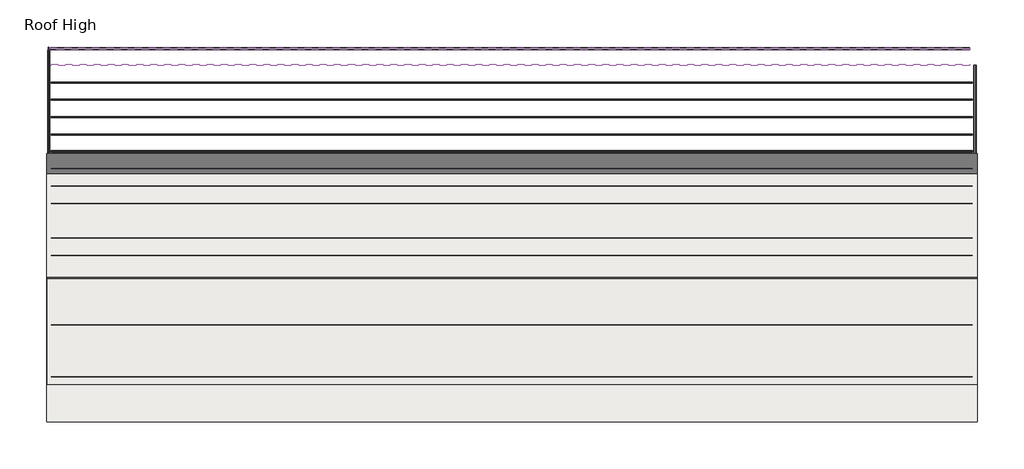
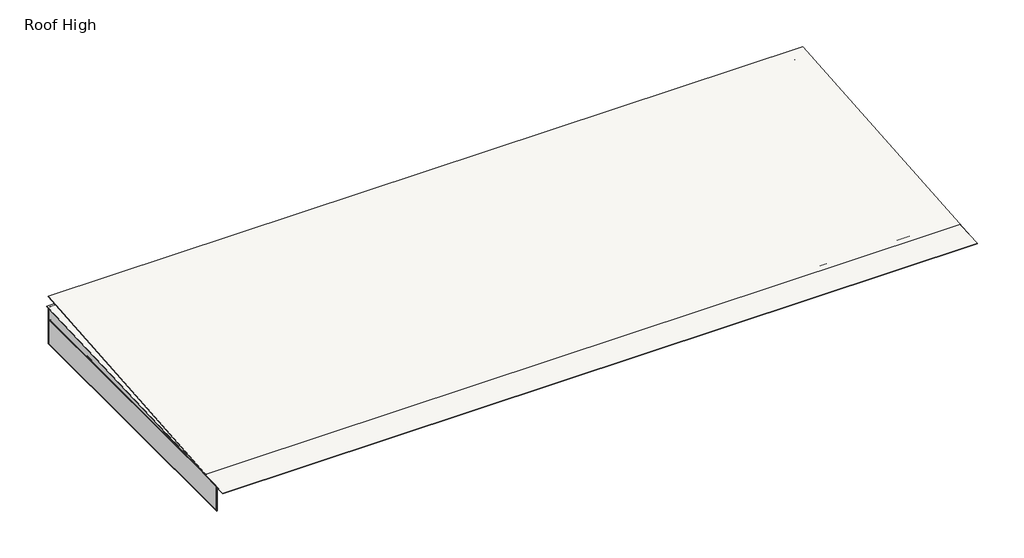
# One storey: 23 beams, 4 members, 2 roofs, 1 plate.
"""IFC4 building model written with IfcOpenShell, lengths in millimetres."""

import ifcopenshell
import ifcopenshell.guid

model = None  # the IFC model being written
_history = None  # IfcOwnerHistory: only IFC2X3 demands one
_inside = {}  # id of a spatial element -> (the spatial element, [elements in it])
_under = {}  # id of a project, library or spatial element -> (it, [spatial elements below it])
_declared = {}  # id of a project -> (the project, [libraries it declares])
_typed = {}  # id of a type object -> (the type object, [elements of that type])
_made_of = {}  # id of a material, layer set ... -> (it, [elements and type objects made of it])


def new_model(schema):
    """Start an empty IFC model of exactly this schema.

    Asked for "IFC4X3", IfcOpenShell would pick the latest addendum, in which some entities
    have other attributes; the version numbers below select the first issue.
    IFC2X3 requires an IfcOwnerHistory on every rooted entity: one is made here for all.
    """
    global model, _history
    if schema == "IFC4X3":
        model = ifcopenshell.file(schema_version=(4, 3, 0, 0))
    else:
        model = ifcopenshell.file(schema=schema)
    _inside.clear()
    _under.clear()
    _declared.clear()
    _typed.clear()
    _made_of.clear()
    _history = None
    if model.schema == "IFC2X3":
        org = make("IfcOrganization", Name="unknown")
        user = make(
            "IfcPersonAndOrganization",
            ThePerson=make("IfcPerson", FamilyName="unknown"),
            TheOrganization=org,
        )
        app = make(
            "IfcApplication",
            ApplicationDeveloper=org,
            Version="unknown",
            ApplicationFullName="unknown",
            ApplicationIdentifier="unknown",
        )
        _history = make(
            "IfcOwnerHistory",
            OwningUser=user,
            OwningApplication=app,
            ChangeAction="ADDED",
            CreationDate=0,
        )
    return model


def make(cls, **values):
    """One entity of the class cls with the attributes given. An attribute that is None is left unset."""
    return model.create_entity(
        cls, **{name: value for name, value in values.items() if value is not None}
    )


def rooted(cls, **values):
    """An entity with a GlobalId (a new one), such as an element, a storey or a relation."""
    return make(cls, GlobalId=ifcopenshell.guid.new(), OwnerHistory=_history, **values)


def si_unit(unit_type, name, prefix=None):
    """IfcSIUnit, for example si_unit("LENGTHUNIT", "METRE", prefix="MILLI")."""
    return make("IfcSIUnit", UnitType=unit_type, Prefix=prefix, Name=name)


def assignment(units):
    """IfcUnitAssignment: the units of a project."""
    return None if units is None else make("IfcUnitAssignment", Units=units)


def point(xyz):
    """IfcCartesianPoint."""
    return None if xyz is None else make("IfcCartesianPoint", Coordinates=xyz)


def direction(xyz):
    """IfcDirection."""
    return None if xyz is None else make("IfcDirection", DirectionRatios=xyz)


def frame(location, z_axis=None, x_axis=None):
    """IfcAxis2Placement3D, a coordinate frame: its origin and axes. An axis left out is left unset."""
    return make(
        "IfcAxis2Placement3D",
        Location=point(location),
        Axis=direction(z_axis),
        RefDirection=direction(x_axis),
    )


def frame_2d(location, x_axis=None):
    """IfcAxis2Placement2D, a coordinate frame in the plane: its origin and x axis."""
    return make(
        "IfcAxis2Placement2D", Location=point(location), RefDirection=direction(x_axis)
    )


def origin():
    """The frame at (0, 0, 0) with its axes left unset."""
    return frame((0.0, 0.0, 0.0))


def place(relative_to, where):
    """IfcLocalPlacement: puts the frame where relative to a parent placement (None: the world)."""
    return make(
        "IfcLocalPlacement", PlacementRelTo=relative_to, RelativePlacement=where
    )


def context(
    kind, dimensions, precision=None, world=None, true_north=None, identifier=None
):
    """IfcGeometricRepresentationContext, for example the 3D "Model" context."""
    return make(
        "IfcGeometricRepresentationContext",
        ContextIdentifier=identifier,
        ContextType=kind,
        CoordinateSpaceDimension=dimensions,
        Precision=precision,
        WorldCoordinateSystem=world,
        TrueNorth=true_north,
    )


def project(units=None, contexts=None):
    """IfcProject with its units and contexts."""
    return rooted(
        "IfcProject",
        Name="project",
        RepresentationContexts=contexts,
        UnitsInContext=assignment(units),
    )


def spatial(cls, under=None, at=None, **own):
    """A site, building, storey or space (cls), placed at a placement, below another one or the project."""
    s = rooted(cls, ObjectPlacement=at, **own)
    if under is not None:
        _under.setdefault(under.id(), (under, []))[1].append(s)
    return s


def polyline(points):
    """IfcPolyline through the points."""
    return make("IfcPolyline", Points=[point(p) for p in points])


def circle_curve(where, radius):
    """IfcCircle in the frame where."""
    return make("IfcCircle", Position=where, Radius=radius)


def trimmed(basis, trim1, trim2, sense, master):
    """IfcTrimmedCurve: the piece of a basis curve between two trims."""
    return make(
        "IfcTrimmedCurve",
        BasisCurve=basis,
        Trim1=trim1,
        Trim2=trim2,
        SenseAgreement=sense,
        MasterRepresentation=master,
    )


def segment(curve, same_sense, transition):
    """IfcCompositeCurveSegment."""
    return make(
        "IfcCompositeCurveSegment",
        Transition=transition,
        SameSense=same_sense,
        ParentCurve=curve,
    )


def composite_curve(segments, self_intersect=None):
    """IfcCompositeCurve: segments joined end to end."""
    return make("IfcCompositeCurve", Segments=segments, SelfIntersect=self_intersect)


def outline(outer, holes=None, kind="AREA"):
    """IfcArbitraryClosedProfileDef: a profile drawn as a closed curve; with holes, ...WithVoids."""
    if holes is None:
        return make("IfcArbitraryClosedProfileDef", ProfileType=kind, OuterCurve=outer)
    return make(
        "IfcArbitraryProfileDefWithVoids",
        ProfileType=kind,
        OuterCurve=outer,
        InnerCurves=holes,
    )


def extrude(swept, where, along, depth):
    """IfcExtrudedAreaSolid: the profile swept, set in the frame where, extruded along a direction by depth."""
    return make(
        "IfcExtrudedAreaSolid",
        SweptArea=swept,
        Position=where,
        ExtrudedDirection=direction(along),
        Depth=depth,
    )


def faces_of(points, faces, orient=None, outer=None):
    """IfcFace entities. A face is a list of loops; a loop is a list of indices into points, from 0.

    orient and outer hold one flag for each loop. By default every Orientation is true, the
    first loop of a face is its IfcFaceOuterBound and the others are IfcFaceBound.
    """
    made = []
    for i, loops in enumerate(faces):
        bounds = []
        for j, loop in enumerate(loops):
            is_outer = j == 0 if outer is None else outer[i][j]
            bounds.append(
                make(
                    "IfcFaceOuterBound" if is_outer else "IfcFaceBound",
                    Bound=make("IfcPolyLoop", Polygon=[points[k] for k in loop]),
                    Orientation=True if orient is None else orient[i][j],
                )
            )
        made.append(make("IfcFace", Bounds=bounds))
    return made


def faceted_brep(points, faces, orient=None, outer=None, voids=None):
    """IfcFacetedBrep: a solid bounded by flat faces; with voids (closed shells), ...WithVoids."""
    shared = [point(p) for p in points]
    hull = make("IfcClosedShell", CfsFaces=faces_of(shared, faces, orient, outer))
    if voids is None:
        return make("IfcFacetedBrep", Outer=hull)
    return make(
        "IfcFacetedBrepWithVoids",
        Outer=hull,
        Voids=[
            make(cls, CfsFaces=faces_of(shared, fs, o, b)) for cls, fs, o, b in voids
        ],
    )


def shape(context_of_items, identifier, shape_type, items):
    """IfcShapeRepresentation: the items that make up one representation, for example the "Body"."""
    return make(
        "IfcShapeRepresentation",
        ContextOfItems=context_of_items,
        RepresentationIdentifier=identifier,
        RepresentationType=shape_type,
        Items=items,
    )


def source(mapping_origin, context_of_items, identifier, shape_type, items):
    """IfcRepresentationMap: a shape defined once, which mapped items show again and again."""
    return make(
        "IfcRepresentationMap",
        MappingOrigin=mapping_origin,
        MappedRepresentation=shape(context_of_items, identifier, shape_type, items),
    )


def transform(
    local_origin,
    x_axis=None,
    y_axis=None,
    z_axis=None,
    scale=None,
    scale2=None,
    scale3=None,
    uniform=True,
):
    """IfcCartesianTransformationOperator3D, or its non-uniform kind. x_axis, y_axis, z_axis: its Axis1, 2, 3."""
    if uniform:
        return make(
            "IfcCartesianTransformationOperator3D",
            Axis1=direction(x_axis),
            Axis2=direction(y_axis),
            LocalOrigin=point(local_origin),
            Scale=scale,
            Axis3=direction(z_axis),
        )
    return make(
        "IfcCartesianTransformationOperator3DnonUniform",
        Axis1=direction(x_axis),
        Axis2=direction(y_axis),
        LocalOrigin=point(local_origin),
        Scale=scale,
        Axis3=direction(z_axis),
        Scale2=scale2,
        Scale3=scale3,
    )


def mapped(mapping_source, mapping_target):
    """IfcMappedItem: shows the shape of a source again, moved by a transform."""
    return make(
        "IfcMappedItem", MappingSource=mapping_source, MappingTarget=mapping_target
    )


def made_of(thing, what):
    """Note that an element or type object is made of a material, layer set ...; save() writes the relation."""
    if what is not None:
        _made_of.setdefault(what.id(), (what, []))[1].append(thing)
    return thing


def element(
    cls,
    number,
    at=None,
    inside=None,
    cuts=None,
    type_object=None,
    material=None,
    context=None,
    identifier="Body",
    shape_type=None,
    held_by="IfcProductDefinitionShape",
    body=None,
    shapes=None,
    **own,
):
    """One element of the class cls, such as IfcWall. Its Tag is "e" and its number.

    at: its placement. inside: the storey or other place that contains it. cuts: it is an
    opening in that element (IfcRelVoidsElement). A single representation is given by context,
    identifier, shape_type and body (its items); several are given by shapes. held_by: the class
    of the entity that holds the representations. save() writes the other relations.
    """
    e = rooted(cls, Tag="e%d" % number, ObjectPlacement=at, **own)
    if body is not None:
        shapes = [shape(context, identifier, shape_type, body)]
    if shapes is not None:
        e.Representation = make(held_by, Representations=shapes)
    if inside is not None:
        _inside.setdefault(inside.id(), (inside, []))[1].append(e)
    if cuts is not None:
        rooted(
            "IfcRelVoidsElement", RelatingBuildingElement=cuts, RelatedOpeningElement=e
        )
    if type_object is not None:
        _typed.setdefault(type_object.id(), (type_object, []))[1].append(e)
    return made_of(e, material)


def aggregate(whole, parts):
    """IfcRelAggregates: a whole, such as a stair, and the parts it consists of."""
    return rooted("IfcRelAggregates", RelatingObject=whole, RelatedObjects=parts)


def save(model, path):
    """Write the relations noted so far, then the file.

    IfcRelAggregates (storeys below a building ...), IfcRelContainedInSpatialStructure (elements
    in a storey), IfcRelDefinesByType, IfcRelAssociatesMaterial and IfcRelDeclares: one each for
    every whole, place, type object, material and project.
    """
    for whole, parts in _under.values():
        aggregate(whole, parts)
    for where, things in _inside.values():
        rooted(
            "IfcRelContainedInSpatialStructure",
            RelatedElements=things,
            RelatingStructure=where,
        )
    for kind, things in _typed.values():
        rooted("IfcRelDefinesByType", RelatedObjects=things, RelatingType=kind)
    for what, things in _made_of.values():
        rooted("IfcRelAssociatesMaterial", RelatedObjects=things, RelatingMaterial=what)
    for by, libraries in _declared.values():
        rooted("IfcRelDeclares", RelatingContext=by, RelatedDefinitions=libraries)
    model.write(path)


def beam_628135af(model_context):
    return source(origin(), model_context, "Body", "SweptSolid", [
        extrude(outline(composite_curve([segment(polyline([(63.5, 127.0), (75.745104, 112.4068534), (73.6169367, 110.621109), (62.204539, 124.221875), (3.3005807, 124.221875)]), True, "CONTINUOUS"), segment(trimmed(circle_curve(frame_2d((3.3741066, 122.2381931)), 1.9850441), [point((3.3005807, 124.221875))], [point((1.3890625, 122.2381931))], True, "CARTESIAN"), True, "CONTINUOUS"), segment(polyline([(1.3890625, 122.2381931), (1.3890625, -122.2375)]), True, "CONTINUOUS"), segment(trimmed(circle_curve(frame_2d((-3.3734375, -122.2375)), 4.7625), [point((1.3890625, -122.2375))], [point((-3.3734375, -127.0))], False, "CARTESIAN"), True, "CONTINUOUS"), segment(polyline([(-3.3734375, -127.0), (-63.5, -127.0), (-75.745104, -112.4068534), (-73.6169367, -110.621109), (-62.204539, -124.221875), (-3.2694106, -124.221875)]), True, "CONTINUOUS"), segment(trimmed(circle_curve(frame_2d((-3.3748024, -122.2389339)), 1.9857399), [point((-3.2694106, -124.221875))], [point((-1.3890625, -122.2389339))], True, "CARTESIAN"), True, "CONTINUOUS"), segment(polyline([(-1.3890625, -122.2389339), (-1.3890625, 122.2375)]), True, "CONTINUOUS"), segment(trimmed(circle_curve(frame_2d((3.3734375, 122.2375)), 4.7625), [point((-1.3890625, 122.2375))], [point((3.3734375, 127.0))], False, "CARTESIAN"), True, "CONTINUOUS"), segment(polyline([(3.3734375, 127.0), (63.5, 127.0)]), True, "CONTINUOUS")], self_intersect=False)), frame((-40443.15, 0.0, 0.0), z_axis=(1.0, 0.0, 0.0), x_axis=(0.0, 1.0, 0.0)), (0.0, 0.0, 1.0), 80644.9999998),
    ])


def beam_f582a1bf(model_context):
    return source(origin(), model_context, "Body", "SweptSolid", [
        extrude(outline(composite_curve([segment(polyline([(63.5, 127.0), (75.745104, 112.4068534), (73.6169367, 110.621109), (62.204539, 124.221875), (3.3005807, 124.221875)]), True, "CONTINUOUS"), segment(trimmed(circle_curve(frame_2d((3.3741066, 122.2381931)), 1.9850441), [point((3.3005807, 124.221875))], [point((1.3890625, 122.2381931))], True, "CARTESIAN"), True, "CONTINUOUS"), segment(polyline([(1.3890625, 122.2381931), (1.3890625, -122.2375)]), True, "CONTINUOUS"), segment(trimmed(circle_curve(frame_2d((-3.3734375, -122.2375)), 4.7625), [point((1.3890625, -122.2375))], [point((-3.3734375, -127.0))], False, "CARTESIAN"), True, "CONTINUOUS"), segment(polyline([(-3.3734375, -127.0), (-63.5, -127.0), (-75.745104, -112.4068534), (-73.6169367, -110.621109), (-62.204539, -124.221875), (-3.2694106, -124.221875)]), True, "CONTINUOUS"), segment(trimmed(circle_curve(frame_2d((-3.3748024, -122.2389339)), 1.9857399), [point((-3.2694106, -124.221875))], [point((-1.3890625, -122.2389339))], True, "CARTESIAN"), True, "CONTINUOUS"), segment(polyline([(-1.3890625, -122.2389339), (-1.3890625, 122.2375)]), True, "CONTINUOUS"), segment(trimmed(circle_curve(frame_2d((3.3734375, 122.2375)), 4.7625), [point((-1.3890625, 122.2375))], [point((3.3734375, 127.0))], False, "CARTESIAN"), True, "CONTINUOUS"), segment(polyline([(3.3734375, 127.0), (63.5, 127.0)]), True, "CONTINUOUS")], self_intersect=False)), frame((-40443.15, 0.0, 0.0), z_axis=(1.0, 0.0, 0.0), x_axis=(0.0, 1.0, 0.0)), (0.0, 0.0, 1.0), 80886.3),
    ])


def beam_ab3afc21(model_context):
    return source(origin(), model_context, "Body", "SweptSolid", [
        extrude(outline(composite_curve([segment(polyline([(-63.5, 101.6), (-3.3734375, 101.6)]), True, "CONTINUOUS"), segment(trimmed(circle_curve(frame_2d((-3.3734375, 96.8375)), 4.7625), [point((-3.3734375, 101.6))], [point((1.3890625, 96.8375))], False, "CARTESIAN"), True, "CONTINUOUS"), segment(polyline([(1.3890625, 96.8375), (1.3890625, -96.8389339)]), True, "CONTINUOUS"), segment(trimmed(circle_curve(frame_2d((3.3748024, -96.8389339)), 1.9857399), [point((1.3890625, -96.8389339))], [point((3.2694106, -98.821875))], True, "CARTESIAN"), True, "CONTINUOUS"), segment(polyline([(3.2694106, -98.821875), (62.204539, -98.821875), (73.6169367, -85.221109), (75.745104, -87.0068534), (63.5, -101.6), (3.3734375, -101.6)]), True, "CONTINUOUS"), segment(trimmed(circle_curve(frame_2d((3.3734375, -96.8375)), 4.7625), [point((3.3734375, -101.6))], [point((-1.3890625, -96.8375))], False, "CARTESIAN"), True, "CONTINUOUS"), segment(polyline([(-1.3890625, -96.8375), (-1.3890625, 96.8381931)]), True, "CONTINUOUS"), segment(trimmed(circle_curve(frame_2d((-3.3741066, 96.8381931)), 1.9850441), [point((-1.3890625, 96.8381931))], [point((-3.3005807, 98.821875))], True, "CARTESIAN"), True, "CONTINUOUS"), segment(polyline([(-3.3005807, 98.821875), (-62.204539, 98.821875), (-73.6169367, 85.221109), (-75.745104, 87.0068534), (-63.5, 101.6)]), True, "CONTINUOUS")], self_intersect=False)), frame((-40605.744726, 0.0, 0.0), z_axis=(1.0, 0.0, 0.0), x_axis=(0.0, 1.0, 0.0)), (0.0, 0.0, 1.0), 80755.8769525),
    ])


def beam_ca91da87(model_context):
    return source(origin(), model_context, "Body", "SweptSolid", [
        extrude(outline(composite_curve([segment(polyline([(-63.5, 101.6), (-3.3734375, 101.6)]), True, "CONTINUOUS"), segment(trimmed(circle_curve(frame_2d((-3.3734375, 96.8375)), 4.7625), [point((-3.3734375, 101.6))], [point((1.3890625, 96.8375))], False, "CARTESIAN"), True, "CONTINUOUS"), segment(polyline([(1.3890625, 96.8375), (1.3890625, -96.8389339)]), True, "CONTINUOUS"), segment(trimmed(circle_curve(frame_2d((3.3748024, -96.8389339)), 1.9857399), [point((1.3890625, -96.8389339))], [point((3.2694106, -98.821875))], True, "CARTESIAN"), True, "CONTINUOUS"), segment(polyline([(3.2694106, -98.821875), (62.204539, -98.821875), (73.6169367, -85.221109), (75.745104, -87.0068534), (63.5, -101.6), (3.3734375, -101.6)]), True, "CONTINUOUS"), segment(trimmed(circle_curve(frame_2d((3.3734375, -96.8375)), 4.7625), [point((3.3734375, -101.6))], [point((-1.3890625, -96.8375))], False, "CARTESIAN"), True, "CONTINUOUS"), segment(polyline([(-1.3890625, -96.8375), (-1.3890625, 96.8381931)]), True, "CONTINUOUS"), segment(trimmed(circle_curve(frame_2d((-3.3741066, 96.8381931)), 1.9850441), [point((-1.3890625, 96.8381931))], [point((-3.3005807, 98.821875))], True, "CARTESIAN"), True, "CONTINUOUS"), segment(polyline([(-3.3005807, 98.821875), (-62.204539, 98.821875), (-73.6169367, 85.221109), (-75.745104, 87.0068534), (-63.5, 101.6)]), True, "CONTINUOUS")], self_intersect=False)), frame((-15624.175, 0.0, 0.0), z_axis=(1.0, 0.0, 0.0), x_axis=(0.0, 1.0, 0.0)), (0.0, 0.0, 1.0), 31235.6499994),
    ])


def beam_e2549a39(model_context):
    return source(origin(), model_context, "Body", "SweptSolid", [
        extrude(outline(composite_curve([segment(polyline([(63.5, 101.6), (75.745104, 87.0068534), (73.6169367, 85.221109), (62.204539, 98.821875), (3.3005807, 98.821875)]), True, "CONTINUOUS"), segment(trimmed(circle_curve(frame_2d((3.3741066, 96.8381931)), 1.9850441), [point((3.3005807, 98.821875))], [point((1.3890625, 96.8381931))], True, "CARTESIAN"), True, "CONTINUOUS"), segment(polyline([(1.3890625, 96.8381931), (1.3890625, -96.8375)]), True, "CONTINUOUS"), segment(trimmed(circle_curve(frame_2d((-3.3734375, -96.8375)), 4.7625), [point((1.3890625, -96.8375))], [point((-3.3734375, -101.6))], False, "CARTESIAN"), True, "CONTINUOUS"), segment(polyline([(-3.3734375, -101.6), (-63.5, -101.6), (-75.745104, -87.0068534), (-73.6169367, -85.221109), (-62.204539, -98.821875), (-3.2694106, -98.821875)]), True, "CONTINUOUS"), segment(trimmed(circle_curve(frame_2d((-3.3748024, -96.8389339)), 1.9857399), [point((-3.2694106, -98.821875))], [point((-1.3890625, -96.8389339))], True, "CARTESIAN"), True, "CONTINUOUS"), segment(polyline([(-1.3890625, -96.8389339), (-1.3890625, 96.8375)]), True, "CONTINUOUS"), segment(trimmed(circle_curve(frame_2d((3.3734375, 96.8375)), 4.7625), [point((-1.3890625, 96.8375))], [point((3.3734375, 101.6))], False, "CARTESIAN"), True, "CONTINUOUS"), segment(polyline([(3.3734375, 101.6), (63.5, 101.6)]), True, "CONTINUOUS")], self_intersect=False)), frame((-15595.6, 0.0, 0.0), z_axis=(1.0, 0.0, 0.0), x_axis=(0.0, 1.0, 0.0)), (0.0, 0.0, 1.0), 29895.5150467),
    ])


def beam_85d20922(model_context):
    return source(origin(), model_context, "Body", "SweptSolid", [
        extrude(outline(composite_curve([segment(polyline([(-63.5, 101.6), (-3.3734375, 101.6)]), True, "CONTINUOUS"), segment(trimmed(circle_curve(frame_2d((-3.3734375, 96.8375)), 4.7625), [point((-3.3734375, 101.6))], [point((1.3890625, 96.8375))], False, "CARTESIAN"), True, "CONTINUOUS"), segment(polyline([(1.3890625, 96.8375), (1.3890625, -96.8389339)]), True, "CONTINUOUS"), segment(trimmed(circle_curve(frame_2d((3.3748024, -96.8389339)), 1.9857399), [point((1.3890625, -96.8389339))], [point((3.2694106, -98.821875))], True, "CARTESIAN"), True, "CONTINUOUS"), segment(polyline([(3.2694106, -98.821875), (62.204539, -98.821875), (73.6169367, -85.221109), (75.745104, -87.0068534), (63.5, -101.6), (3.3734375, -101.6)]), True, "CONTINUOUS"), segment(trimmed(circle_curve(frame_2d((3.3734375, -96.8375)), 4.7625), [point((3.3734375, -101.6))], [point((-1.3890625, -96.8375))], False, "CARTESIAN"), True, "CONTINUOUS"), segment(polyline([(-1.3890625, -96.8375), (-1.3890625, 96.8381931)]), True, "CONTINUOUS"), segment(trimmed(circle_curve(frame_2d((-3.3741066, 96.8381931)), 1.9850441), [point((-1.3890625, 96.8381931))], [point((-3.3005807, 98.821875))], True, "CARTESIAN"), True, "CONTINUOUS"), segment(polyline([(-3.3005807, 98.821875), (-62.204539, 98.821875), (-73.6169367, 85.221109), (-75.745104, 87.0068534), (-63.5, 101.6)]), True, "CONTINUOUS")], self_intersect=False)), frame((-40618.4447266, 0.0, 0.0), z_axis=(1.0, 0.0, 0.0), x_axis=(0.0, 1.0, 0.0)), (0.0, 0.0, 1.0), 80768.5769531),
    ])


def rectangular_mullion_profile_polycarbonate_lower_9942ed0a(model_context):
    return source(origin(), model_context, "Body", "SweptSolid", [
        extrude(outline(polyline([(0.0, -28.984575), (-56.9976, -28.984575), (-56.9976, -19.992975), (-50.6476, -19.992975), (-50.6476, -21.580475), (-55.4101, -21.580475), (-55.4101, -27.397075), (-1.5875, -27.397075), (-1.5875, 23.428325), (-35.3949, 23.428325), (-35.3949, 21.840825), (-36.9824, 21.840825), (-36.9824, 25.015825), (0.0, 25.015825), (0.0, -28.984575)])), frame((0.0, 0.0, -31440.30288), z_axis=(0.0, 0.0, 1.0), x_axis=(1.0, 0.0, 0.0)), (0.0, 0.0, 1.0), 31440.30288),
    ])


def rectangular_mullion_profile_polycarbonate_upper_and_left_a248562a(model_context):
    return source(origin(), model_context, "Body", "Brep", [
        faceted_brep([(0.0, 25.015825, 0.0), (0.0, -28.984575, 0.0), (0.0, -28.984575, -31651.7402253), (0.0, 25.015825, -31651.7402253), (-71.9836, 25.015825, -69.046742), (-71.9836, 25.015825, -31576.6948499), (-71.9836, 21.840825, -69.046742), (-71.9836, 21.840825, -31576.6948499), (-70.3961, 21.840825, -67.5240104), (-70.3961, 21.840825, -31578.3498732), (-70.3961, 23.428325, -67.5240104), (-70.3961, 23.428325, -31578.3498732), (-1.5875, 23.428325, -1.5227316), (-1.5875, 23.428325, -31650.085202), (-1.5875, -27.397075, -1.5227316), (-1.5875, -27.397075, -31650.085202), (-90.4113, -27.397075, -86.7226105), (-90.4113, -27.397075, -31557.4833398), (-90.4113, -21.580475, -86.7226105), (-90.4113, -21.580475, -31557.4833398), (-85.6488, -21.580475, -82.1544157), (-85.6488, -21.580475, -31562.4484096), (-85.6488, -19.992975, -82.1544157), (-85.6488, -19.992975, -31562.4484096), (-91.9988, -19.992975, -88.2453421), (-91.9988, -19.992975, -31555.8283165), (-91.9988, -28.984575, -88.2453421), (-91.9988, -28.984575, -31555.8283165)], [[[0, 1, 2, 3]], [[4, 0, 3, 5]], [[6, 4, 5, 7]], [[8, 6, 7, 9]], [[10, 8, 9, 11]], [[12, 10, 11, 13]], [[14, 12, 13, 15]], [[16, 14, 15, 17]], [[18, 16, 17, 19]], [[20, 18, 19, 21]], [[22, 20, 21, 23]], [[24, 22, 23, 25]], [[26, 24, 25, 27]], [[1, 26, 27, 2]], [[1, 0, 4, 6, 8, 10, 12, 14, 16, 18, 20, 22, 24, 26]], [[2, 27, 25, 23, 21, 19, 17, 15, 13, 11, 9, 7, 5, 3]]]),
    ])


def rectangular_mullion_profile_polycarbonate_upper_and_left_c928ab11(model_context):
    return source(origin(), model_context, "Body", "Brep", [
        faceted_brep([(0.0, -28.984575, 0.0), (0.0, 25.015825, 0.0), (-71.9836, 25.015825, 0.0), (-71.9836, 21.840825, 0.0), (-70.3961, 21.840825, 0.0), (-70.3961, 23.428325, 0.0), (-1.5875, 23.428325, 0.0), (-1.5875, -27.397075, 0.0), (-90.4113, -27.397075, 0.0), (-90.4113, -21.580475, 0.0), (-85.6488, -21.580475, 0.0), (-85.6488, -19.992975, 0.0), (-91.9988, -19.992975, 0.0), (-91.9988, -28.984575, 0.0), (0.0, -28.984575, -2875.2880888), (0.0, 25.015825, -2875.2880888), (-71.9836, 25.015825, -2806.2413468), (-71.9836, 21.840825, -2806.2413468), (-70.3961, 21.840825, -2807.7640784), (-70.3961, 23.428325, -2807.7640784), (-1.5875, 23.428325, -2873.7653572), (-1.5875, -27.397075, -2873.7653572), (-90.4113, -27.397075, -2788.5654783), (-90.4113, -21.580475, -2788.5654783), (-85.6488, -21.580475, -2793.1336732), (-85.6488, -19.992975, -2793.1336732), (-91.9988, -19.992975, -2787.0427467), (-91.9988, -28.984575, -2787.0427467)], [[[0, 1, 2, 3, 4, 5, 6, 7, 8, 9, 10, 11, 12, 13]], [[1, 0, 14, 15]], [[2, 1, 15, 16]], [[3, 2, 16, 17]], [[4, 3, 17, 18]], [[5, 4, 18, 19]], [[6, 5, 19, 20]], [[7, 6, 20, 21]], [[8, 7, 21, 22]], [[9, 8, 22, 23]], [[10, 9, 23, 24]], [[11, 10, 24, 25]], [[12, 11, 25, 26]], [[13, 12, 26, 27]], [[0, 13, 27, 14]], [[14, 27, 26, 25, 24, 23, 22, 21, 20, 19, 18, 17, 16, 15]]]),
    ])


def rectangular_mullion_profile_polycarbonate_right_c7f88d5a(model_context):
    return source(origin(), model_context, "Body", "Brep", [
        faceted_brep([(0.0, -28.984575, -4192.9672755), (-91.9988, -28.984575, -4192.9672755), (-91.9988, -19.992975, -4192.9672755), (-85.6488, -19.992975, -4192.9672755), (-85.6488, -21.580475, -4192.9672755), (-90.4113, -21.580475, -4192.9672755), (-90.4113, -27.397075, -4192.9672755), (-1.5875, -27.397075, -4192.9672755), (-1.5875, 23.428325, -4192.9672755), (-70.3961, 23.428325, -4192.9672755), (-70.3961, 21.840825, -4192.9672755), (-71.9836, 21.840825, -4192.9672755), (-71.9836, 25.015825, -4192.9672755), (0.0, 25.015825, -4192.9672755), (0.0, 25.015825, 0.0), (0.0, -28.984575, 0.0), (-71.9836, 25.015825, -75.0453753), (-71.9836, 21.840825, -75.0453753), (-70.3961, 21.840825, -73.3903521), (-70.3961, 23.428325, -73.3903521), (-1.5875, 23.428325, -1.6550233), (-1.5875, -27.397075, -1.6550233), (-90.4113, -27.397075, -94.2568855), (-90.4113, -21.580475, -94.2568855), (-85.6488, -21.580475, -89.2918157), (-85.6488, -19.992975, -89.2918157), (-91.9988, -19.992975, -95.9119088), (-91.9988, -28.984575, -95.9119088)], [[[0, 1, 2, 3, 4, 5, 6, 7, 8, 9, 10, 11, 12, 13]], [[14, 15, 0, 13]], [[16, 14, 13, 12]], [[17, 16, 12, 11]], [[18, 17, 11, 10]], [[19, 18, 10, 9]], [[20, 19, 9, 8]], [[21, 20, 8, 7]], [[22, 21, 7, 6]], [[23, 22, 6, 5]], [[24, 23, 5, 4]], [[25, 24, 4, 3]], [[26, 25, 3, 2]], [[27, 26, 2, 1]], [[15, 27, 1, 0]], [[15, 14, 16, 17, 18, 19, 20, 21, 22, 23, 24, 25, 26, 27]]]),
    ])


model = new_model("IFC4")

# Units and contexts
model_context = context("Model", 3, world=origin())
ifc_project = project(units=[si_unit("LENGTHUNIT", "METRE", prefix="MILLI")], contexts=[model_context])

# Site, building, storey
site = spatial("IfcSite", under=ifc_project)
building = spatial("IfcBuilding", under=site)
storey = spatial("IfcBuildingStorey", under=building, Name="Roof High", Elevation=8352.1898378)

# Beams
placement = place(None, origin())
beam_shape = beam_628135af(model_context)
element("IfcBeam", 1, ObjectType="Girt_Z : 10\"D", at=placement, inside=storey, context=model_context, shape_type="MappedRepresentation", body=[
    mapped(beam_shape, transform((619471.4617241, -538117.5418931, 9711.5416785), x_axis=(1.0, 0.0, 0.0), y_axis=(0.0, 0.9991330730923521, 0.04163054471217894), z_axis=(0.0, -0.04163054471217894, 0.9991330730923521))),
])
beam_2_shape = beam_f582a1bf(model_context)
element("IfcBeam", 2, ObjectType="Girt_Z : 10\"D", at=placement, inside=storey, context=model_context, shape_type="MappedRepresentation", body=[
    mapped(beam_2_shape, transform((619471.4617241, -539640.2206965, 9648.0967284), x_axis=(1.0, 0.0, 0.0), y_axis=(0.0, 0.9991330730923521, 0.04163054471217894), z_axis=(0.0, -0.04163054471217894, 0.9991330730923521))),
])
element("IfcBeam", 3, ObjectType="Girt_Z : 10\"D", at=placement, inside=storey, context=model_context, shape_type="MappedRepresentation", body=[
    mapped(beam_2_shape, transform((619471.4617241, -541162.8994999, 9584.6517782), x_axis=(1.0, 0.0, 0.0), y_axis=(0.0, 0.9991330730923521, 0.04163054471217894), z_axis=(0.0, -0.04163054471217894, 0.9991330730923521))),
])
element("IfcBeam", 4, ObjectType="Girt_Z : 10\"D", at=placement, inside=storey, context=model_context, shape_type="MappedRepresentation", body=[
    mapped(beam_2_shape, transform((619471.4617241, -542685.5783033, 9521.2068281), x_axis=(1.0, 0.0, 0.0), y_axis=(0.0, 0.9991330730923521, 0.04163054471217894), z_axis=(0.0, -0.04163054471217894, 0.9991330730923521))),
])
element("IfcBeam", 5, ObjectType="Girt_Z : 10\"D", at=placement, inside=storey, context=model_context, shape_type="MappedRepresentation", body=[
    mapped(beam_2_shape, transform((619471.4617241, -544208.2571067, 9457.7618779), x_axis=(1.0, 0.0, 0.0), y_axis=(0.0, 0.9991330730923521, 0.04163054471217894), z_axis=(0.0, -0.04163054471217894, 0.9991330730923521))),
])
element("IfcBeam", 6, ObjectType="Girt_Z : 10\"D", at=placement, inside=storey, context=model_context, shape_type="MappedRepresentation", body=[
    mapped(beam_2_shape, transform((619471.4617241, -545730.93591, 9394.3169278), x_axis=(1.0, 0.0, 0.0), y_axis=(0.0, 0.9991330730923521, 0.04163054471217894), z_axis=(0.0, -0.04163054471217894, 0.9991330730923521))),
])
element("IfcBeam", 7, ObjectType="Girt_Z : 10\"D", at=placement, inside=storey, context=model_context, shape_type="MappedRepresentation", body=[
    mapped(beam_2_shape, transform((619471.4617241, -547253.6147134, 9330.8719777), x_axis=(1.0, 0.0, 0.0), y_axis=(0.0, 0.9991330730923521, 0.04163054471217894), z_axis=(0.0, -0.04163054471217894, 0.9991330730923521))),
])
element("IfcBeam", 8, ObjectType="Girt_Z : 10\"D", at=placement, inside=storey, context=model_context, shape_type="MappedRepresentation", body=[
    mapped(beam_2_shape, transform((619471.4617241, -548776.2935168, 9267.4270275), x_axis=(1.0, 0.0, 0.0), y_axis=(0.0, 0.9991330730923521, 0.04163054471217894), z_axis=(0.0, -0.04163054471217894, 0.9991330730923521))),
])
element("IfcBeam", 9, ObjectType="Girt_Z : 10\"D", at=placement, inside=storey, context=model_context, shape_type="MappedRepresentation", body=[
    mapped(beam_2_shape, transform((619471.4617241, -550298.9723202, 9203.9820774), x_axis=(1.0, 0.0, 0.0), y_axis=(0.0, 0.9991330730923521, 0.04163054471217894), z_axis=(0.0, -0.04163054471217894, 0.9991330730923521))),
])
element("IfcBeam", 10, ObjectType="Girt_Z : 10\"D", at=placement, inside=storey, context=model_context, shape_type="MappedRepresentation", body=[
    mapped(beam_2_shape, transform((619471.4617241, -551821.6511236, 9140.5371272), x_axis=(1.0, 0.0, 0.0), y_axis=(0.0, 0.9991330730923521, 0.04163054471217894), z_axis=(0.0, -0.04163054471217894, 0.9991330730923521))),
])
element("IfcBeam", 11, ObjectType="Girt_Z : 10\"D", at=placement, inside=storey, context=model_context, shape_type="MappedRepresentation", body=[
    mapped(beam_2_shape, transform((619471.4617241, -553344.329927, 9077.0921771), x_axis=(1.0, 0.0, 0.0), y_axis=(0.0, 0.9991330730923521, 0.04163054471217894), z_axis=(0.0, -0.04163054471217894, 0.9991330730923521))),
])
element("IfcBeam", 12, ObjectType="Girt_Z : 10\"D", at=placement, inside=storey, context=model_context, shape_type="MappedRepresentation", body=[
    mapped(beam_2_shape, transform((619471.4617241, -554867.0087304, 9013.647227), x_axis=(1.0, 0.0, 0.0), y_axis=(0.0, 0.9991330730923521, 0.04163054471217894), z_axis=(0.0, -0.04163054471217894, 0.9991330730923521))),
])
element("IfcBeam", 13, ObjectType="Girt_Z : 10\"D", at=placement, inside=storey, context=model_context, shape_type="MappedRepresentation", body=[
    mapped(beam_2_shape, transform((619471.4617241, -556389.6875338, 8950.2022768), x_axis=(1.0, 0.0, 0.0), y_axis=(0.0, 0.9991330730923521, 0.04163054471217894), z_axis=(0.0, -0.04163054471217894, 0.9991330730923521))),
])
element("IfcBeam", 14, ObjectType="Girt_Z : 10\"D", at=placement, inside=storey, context=model_context, shape_type="MappedRepresentation", body=[
    mapped(beam_2_shape, transform((619471.4617241, -557912.3663372, 8886.7573267), x_axis=(1.0, 0.0, 0.0), y_axis=(0.0, 0.9991330730923521, 0.04163054471217894), z_axis=(0.0, -0.04163054471217894, 0.9991330730923521))),
])
element("IfcBeam", 15, ObjectType="Girt_Z : 10\"D", at=placement, inside=storey, context=model_context, shape_type="MappedRepresentation", body=[
    mapped(beam_2_shape, transform((619471.4617241, -559435.0451406, 8823.3123765), x_axis=(1.0, 0.0, 0.0), y_axis=(0.0, 0.9991330730923521, 0.04163054471217894), z_axis=(0.0, -0.04163054471217894, 0.9991330730923521))),
])
element("IfcBeam", 16, ObjectType="Girt_Z : 10\"D", at=placement, inside=storey, context=model_context, shape_type="MappedRepresentation", body=[
    mapped(beam_2_shape, transform((619471.4617241, -560957.723944, 8759.8674264), x_axis=(1.0, 0.0, 0.0), y_axis=(0.0, 0.9991330730923521, 0.04163054471217894), z_axis=(0.0, -0.04163054471217894, 0.9991330730923521))),
])
element("IfcBeam", 17, ObjectType="Girt_Z : 10\"D", at=placement, inside=storey, context=model_context, shape_type="MappedRepresentation", body=[
    mapped(beam_2_shape, transform((619471.4617241, -562480.4027474, 8696.4224762), x_axis=(1.0, 0.0, 0.0), y_axis=(0.0, 0.9991330730923521, 0.04163054471217894), z_axis=(0.0, -0.04163054471217894, 0.9991330730923521))),
])
element("IfcBeam", 18, ObjectType="Girt_Z : 10\"D", at=placement, inside=storey, context=model_context, shape_type="MappedRepresentation", body=[
    mapped(beam_2_shape, transform((619471.4617241, -564003.0815508, 8632.9775261), x_axis=(1.0, 0.0, 0.0), y_axis=(0.0, 0.9991330730923521, 0.04163054471217894), z_axis=(0.0, -0.04163054471217894, 0.9991330730923521))),
])
element("IfcBeam", 19, ObjectType="Girt_Z : 10\"D", at=placement, inside=storey, context=model_context, shape_type="MappedRepresentation", body=[
    mapped(beam_2_shape, transform((619471.4617241, -565525.7603542, 8569.532576), x_axis=(1.0, 0.0, 0.0), y_axis=(0.0, 0.9991330730923521, 0.04163054471217894), z_axis=(0.0, -0.04163054471217894, 0.9991330730923521))),
])
beam_3_shape = beam_ab3afc21(model_context)
element("IfcBeam", 20, ObjectType="Girt_Z : 8\"D", at=placement, inside=storey, context=model_context, shape_type="MappedRepresentation", body=[
    mapped(beam_3_shape, transform((619523.1794974, -536696.9913841, 8585.2), x_axis=(1.0000000000000002, 0.0, 0.0), y_axis=(0.0, 0.0, 1.0000000000000002), z_axis=(0.0, -1.0000000000000002, 0.0))),
])
beam_4_shape = beam_ca91da87(model_context)
element("IfcBeam", 21, ObjectType="Girt_Z : 8\"D", at=placement, inside=storey, context=model_context, shape_type="MappedRepresentation", body=[
    mapped(beam_4_shape, transform((578803.1347708, -552422.7663841, 8585.2), x_axis=(0.0, 1.0000000000000002, 0.0), y_axis=(0.0, 0.0, 1.0000000000000002), z_axis=(1.0000000000000002, 0.0, 0.0))),
])
beam_5_shape = beam_e2549a39(model_context)
element("IfcBeam", 22, ObjectType="Girt_Z : 8\"D", at=placement, inside=storey, context=model_context, shape_type="MappedRepresentation", body=[
    mapped(beam_5_shape, transform((660139.7886771, -552451.3413841, 8585.2), x_axis=(0.0, 1.0000000000000002, 0.0), y_axis=(0.0, 0.0, -1.0000000000000002), z_axis=(-1.0000000000000002, 0.0, 0.0))),
])
beam_6_shape = beam_85d20922(model_context)
element("IfcBeam", 23, ObjectType="Girt_Z : 8\"D", at=placement, inside=storey, context=model_context, shape_type="MappedRepresentation", body=[
    mapped(beam_6_shape, transform((619523.1794974, -536696.9913841, 9810.75), x_axis=(1.0000000000000002, 0.0, 0.0), y_axis=(0.0, 0.0, 1.0000000000000002), z_axis=(0.0, -1.0000000000000002, 0.0))),
])

# Members
rectangular_mullion_profile_polycarbonate_lower_shape = rectangular_mullion_profile_polycarbonate_lower_9942ed0a(model_context)
element("IfcMember", 24, ObjectType="Rectangular Mullion : Profile_Polycarbonate_Lower", at=placement, inside=storey, context=model_context, shape_type="MappedRepresentation", body=[
    mapped(rectangular_mullion_profile_polycarbonate_lower_shape, transform((578786.7847654, -536651.8149441, 5710.5898378), x_axis=(0.0, 0.0, -1.0), y_axis=(-1.0, 0.0, 0.0), z_axis=(0.0, 1.0, 0.0))),
])
rectangular_mullion_profile_polycarbonate_upper_and_left_shape = rectangular_mullion_profile_polycarbonate_upper_and_left_a248562a(model_context)
element("IfcMember", 25, ObjectType="Rectangular Mullion : Profile_Polycarbonate_Upper and left", at=placement, inside=storey, context=model_context, shape_type="MappedRepresentation", body=[
    mapped(rectangular_mullion_profile_polycarbonate_upper_and_left_shape, transform((578786.7847654, -568184.1166241, 8585.8779266), x_axis=(0.0, -0.041630544712178995, 0.9991330730923521), y_axis=(-1.0, 0.0, 0.0), z_axis=(0.0, -0.999133073092352, -0.04163054471217899))),
])
rectangular_mullion_profile_polycarbonate_upper_and_left_2_shape = rectangular_mullion_profile_polycarbonate_upper_and_left_c928ab11(model_context)
element("IfcMember", 26, ObjectType="Rectangular Mullion : Profile_Polycarbonate_Upper and left", at=placement, inside=storey, context=model_context, shape_type="MappedRepresentation", body=[
    mapped(rectangular_mullion_profile_polycarbonate_upper_and_left_2_shape, transform((578786.7847654, -568184.1166241, 5710.5898378), x_axis=(0.0, -1.0, 0.0), y_axis=(-1.0, 0.0, 0.0), z_axis=(0.0, 0.0, -1.0))),
])
rectangular_mullion_profile_polycarbonate_right_shape = rectangular_mullion_profile_polycarbonate_right_c7f88d5a(model_context)
element("IfcMember", 27, ObjectType="Rectangular Mullion : Profile_Polycarbonate_right", at=placement, inside=storey, context=model_context, shape_type="MappedRepresentation", body=[
    mapped(rectangular_mullion_profile_polycarbonate_right_shape, transform((578786.7847654, -536559.8161441, 9903.5571133), x_axis=(0.0, 1.0, 0.0), y_axis=(-1.0, 0.0, 0.0), z_axis=(0.0, 0.0, 1.0))),
])

# Plate
element("IfcPlate", 28, ObjectType="arcoPlus - 547", at=placement, inside=storey, context=model_context, shape_type="SweptSolid", body=[
    extrude(outline(polyline([(-536561.4036441, 5712.1773378), (-568182.5291241, 5712.1773378), (-568182.5291241, 8584.355195), (-536561.4036441, 9901.90209), (-536561.4036441, 5712.1773378)])), frame((578766.7848054, 0.0, 0.0), z_axis=(1.0, 0.0, 0.0), x_axis=(0.0, 1.0, 0.0)), (0.0, 0.0, 1.0), 39.99992),
])

# Roofs
element("IfcRoof", 29, ObjectType="arcoPlus_6124_with_IR", at=placement, inside=storey, context=model_context, shape_type="SweptSolid", body=[
    extrude(outline(polyline([(-568168.5413949, 8617.4506711), (-536724.1414187, 11237.8173358), (-536724.1414187, 11225.7702535), (-568168.5413949, 8605.4035888), (-568168.5413949, 8617.4506711)])), frame((578668.83476, 0.0, 0.0), z_axis=(1.0, 0.0, 0.0), x_axis=(0.0, 1.0, 0.0)), (0.0, 0.0, 1.0), 81697.5769747),
])
element("IfcRoof", 30, ObjectType="Metal Roof - Structural Standing Seam", at=placement, inside=storey, context=model_context, shape_type="SweptSolid", body=[
    extrude(outline(polyline([(-569520.1413841, 8641.3985906), (-536506.4913841, 10016.9673406), (-536506.4913841, 9943.8789783), (-569520.1413841, 8568.3102283), (-569520.1413841, 8641.3985906)])), frame((578612.6347708, 0.0, 0.0), z_axis=(1.0, 0.0, 0.0), x_axis=(0.0, 1.0, 0.0)), (0.0, 0.0, 1.0), 81717.6539063),
])

save(model, "model.ifc")

# Revit data of these elements
# Project information
#   Project Issue Date = "04/07/2015"
#   Project Status = "Project Status"
#   Client Name = "Xcel"
#   Project Address = "Enter address here"
#   Project Name = "Sports Complex"
#   Project Number = "Project Number"
# Grids (mm)
#   "1": line (560645.062, -472874.843) -> (560645.062, -606417.413)
#   "H.5": line (499667.271, -572593.541) -> (746385.635, -572593.541)
#   "2": line (579028.312, -472874.843) -> (579028.312, -606417.413)
#   "3": line (586381.612, -472874.843) -> (586381.612, -606417.413)
#   "4": line (593734.912, -472874.843) -> (593734.912, -606417.413)
#   "5": line (601088.212, -472874.843) -> (601088.212, -606417.413)
#   "6": line (608441.512, -472874.843) -> (608441.512, -606417.413)
#   "7": line (615794.812, -472874.843) -> (615794.812, -606417.413)
#   "8": line (623148.112, -472874.843) -> (623148.112, -606417.413)
#   "9": line (630501.412, -472874.843) -> (630501.412, -606417.413)
#   "10": line (637854.712, -472874.843) -> (637854.712, -606417.413)
#   "11": line (645208.012, -472874.843) -> (645208.012, -606417.413)
#   "12": line (652561.312, -472874.843) -> (652561.312, -606417.413)
#   "13": line (659914.612, -472874.843) -> (659914.612, -606417.413)
#   "B": line (499667.271, -537052.591) -> (746385.635, -537052.591)
#   "G": line (499667.271, -567691.341) -> (746385.635, -567691.341)
#   "H": line (499667.271, -578721.291) -> (746385.635, -578721.291)
#   "14": line (667267.912, -472874.843) -> (667267.912, -606417.413)
#   "A": line (499667.271, -530924.841) -> (746385.635, -530924.841)
#   "C": line (499667.271, -543180.341) -> (682636.572, -543180.341)
#   "D": line (499667.271, -549308.091) -> (682636.572, -549308.091)
#   "E": line (499667.271, -555435.841) -> (682636.572, -555435.841)
#   "F": line (499667.271, -561563.591) -> (682636.572, -561563.591)
# Type "Girt_Z : 10\"D"
#   Web_Thickness = 0' - 0 7/64"
#   Length [instance default] = 10' - 0"
#   Leg_1 = 0' - 2 1/2"
#   Height = 0' - 10"
#   Structural Material [instance default] = none
# Type "Girt_Z : 8\"D"
#   Web_Thickness = 0' - 0 7/64"
#   Length [instance default] = 10' - 0"
#   Leg_1 = 0' - 2 1/2"
#   Height = 0' - 8"
#   Structural Material [instance default] = none
# Type "Rectangular Mullion : Profile_Polycarbonate_Lower"
#   built-in parameter 1007322 = 0.177167 (stored number, unit not read)
#   built-in parameter 1007321 = 0 (stored number, unit not read)
#   built-in parameter 1007320 = 0.00520833 (stored number, unit not read)
# Type "Rectangular Mullion : Profile_Polycarbonate_Upper and left"
#   built-in parameter 1007322 = 0.177167 (stored number, unit not read)
#   built-in parameter 1007321 = 0.00520833 (stored number, unit not read)
#   built-in parameter 1007320 = 0 (stored number, unit not read)
# Type "Rectangular Mullion : Profile_Polycarbonate_right"
#   built-in parameter 1007322 = 0.177167 (stored number, unit not read)
#   built-in parameter 1007321 = 0 (stored number, unit not read)
#   built-in parameter 1007320 = 0.00520833 (stored number, unit not read)
# Type "arcoPlus - 547"
#   Assembly Code = "B2010"
#   Width = 0' - 1.5748"
#   Elevation_Transparency_Hack = 70
#   Layers, outside or top first: 0' - 1 147/256" "arcoPlus_324" (function 1)
# Type "arcoPlus_6124_with_IR"
#   Assembly Code = "B1020"
#   built-in parameter 1001600 = 0.039388 (stored number, unit not read)
#   Elevation_Transparency_Hack = 70
#   Layers, outside or top first: 0' - 0 121/256" "arcoPlus_6124_with_IR" (function 1)
# Type "Metal Roof - Structural Standing Seam"
#   Assembly Code = "B1020"
#   built-in parameter 1001600 = 0.239583 (stored number, unit not read)
#   Elevation_Transparency_Hack = 0
#   Layers, outside or top first: 0' - 2 7/8" "Metal Roof - Structural Standing Seam" (function 1)
# Elements 1, 2, 3, 4, 5, 6, 7, 8, 9, 10, 11, 12, 13, 14, 15, 16, 17, 18, 19 (IfcBeam, "Girt_Z : 10\"D")
#   Structural Material = none
#   Phase Created = Phase 1
# Elements 20, 21, 22, 23 (IfcBeam, "Girt_Z : 8\"D")
#   Comments = ""
#   Structural Material = Steel
#   Structural Material = Steel
#   Phase Created = Phase 1
#   Materials on its faces: "Steel"
# Element 24 (IfcMember, "Rectangular Mullion : Profile_Polycarbonate_Lower")
#   Phase Created = Phase 1
# Elements 25, 26 (IfcMember, "Rectangular Mullion : Profile_Polycarbonate_Upper and left")
#   Phase Created = Phase 1
# Element 27 (IfcMember, "Rectangular Mullion : Profile_Polycarbonate_right")
#   Phase Created = Phase 1
# Element 28 (IfcPlate, "arcoPlus - 547")
#   built-in parameter 1001111 = -8' - 8"
#   Top Offset = 0' - 0"
#   Base Offset = -8' - 8"
#   Unconnected Height = 13' - 9.07745"
#   wall height = 13' - 9.07745"
#   Phase Created = Phase 1
#   Base Constraint = Roof High
#   Materials on its faces: "arcoPlus_324"
# Element 29 (IfcRoof, "arcoPlus_6124_with_IR")
#   OD_Option_2 = "N"
#   OD_Option_3 = "N"
#   OD_Option_4 = "N"
#   built-in parameter 1001705 = 36.8695 (stored number, unit not read)
#   built-in parameter 1001701 = 0.830754 (stored number, unit not read)
#   built-in parameter 1001710 = 33615
#   Phase Created = Phase 1
#   Materials on its faces: "arcoPlus_6124_with_IR"
# Element 30 (IfcRoof, "Metal Roof - Structural Standing Seam")
#   OD_Option_1 = "N"
#   OD_Option_2 = ""
#   OD_Option_3 = "N"
#   OD_Option_4 = "N"
#   built-in parameter 1001705 = 32.8641 (stored number, unit not read)
#   built-in parameter 1001701 = 0.709056 (stored number, unit not read)
#   built-in parameter 1001710 = 33615
#   Phase Created = Phase 1
#   Materials on its faces: "Metal Roof - Structural Standing Seam"
# Materials
#   "arcoPlus_324": class "Miscellaneous", colour RGB 197 197 197, transparency 0.3, Cost = 0
#   "arcoPlus_6124_with_IR": class "Miscellaneous", colour RGB 196 196 196, transparency 0.3, Cost = 0
#   "Metal Roof - Structural Standing Seam": class "Generic", colour RGB 219 219 219, transparency 0, Cost = 0
#   "Steel": class "Metal", colour RGB 118 118 114, transparency 0, Description = "Steel, mill finish", Cost = 0
